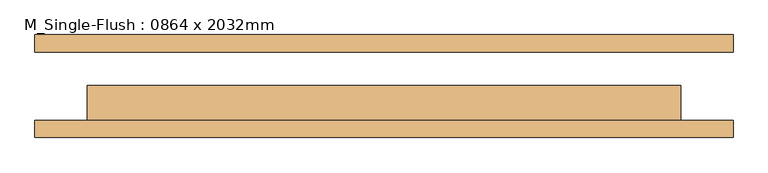
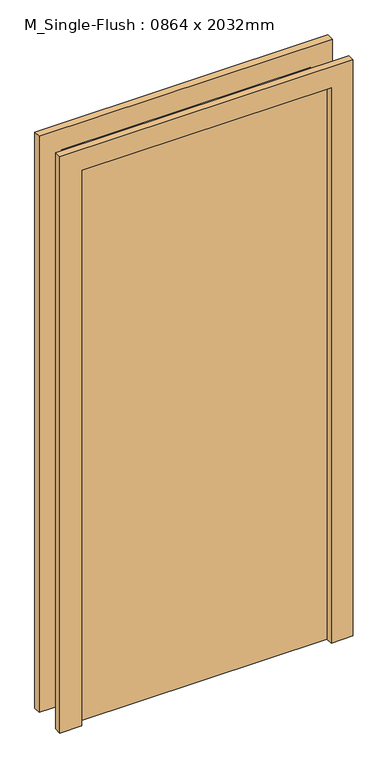
"""IFC4 building model written with IfcOpenShell, lengths in millimetres: door geometry, M_Single-Flush : 0864 x 2032mm."""

import ifcopenshell
import ifcopenshell.guid

model = None  # the IFC model being written
_history = None  # IfcOwnerHistory: only IFC2X3 demands one
_inside = {}  # id of a spatial element -> (the spatial element, [elements in it])
_under = {}  # id of a project, library or spatial element -> (it, [spatial elements below it])
_declared = {}  # id of a project -> (the project, [libraries it declares])
_typed = {}  # id of a type object -> (the type object, [elements of that type])
_made_of = {}  # id of a material, layer set ... -> (it, [elements and type objects made of it])


def new_model(schema):
    """Start an empty IFC model of exactly this schema.

    Asked for "IFC4X3", IfcOpenShell would pick the latest addendum, in which some entities
    have other attributes; the version numbers below select the first issue.
    IFC2X3 requires an IfcOwnerHistory on every rooted entity: one is made here for all.
    """
    global model, _history
    if schema == "IFC4X3":
        model = ifcopenshell.file(schema_version=(4, 3, 0, 0))
    else:
        model = ifcopenshell.file(schema=schema)
    _inside.clear()
    _under.clear()
    _declared.clear()
    _typed.clear()
    _made_of.clear()
    _history = None
    if model.schema == "IFC2X3":
        org = make("IfcOrganization", Name="unknown")
        user = make(
            "IfcPersonAndOrganization",
            ThePerson=make("IfcPerson", FamilyName="unknown"),
            TheOrganization=org,
        )
        app = make(
            "IfcApplication",
            ApplicationDeveloper=org,
            Version="unknown",
            ApplicationFullName="unknown",
            ApplicationIdentifier="unknown",
        )
        _history = make(
            "IfcOwnerHistory",
            OwningUser=user,
            OwningApplication=app,
            ChangeAction="ADDED",
            CreationDate=0,
        )
    return model


def make(cls, **values):
    """One entity of the class cls with the attributes given. An attribute that is None is left unset."""
    return model.create_entity(
        cls, **{name: value for name, value in values.items() if value is not None}
    )


def rooted(cls, **values):
    """An entity with a GlobalId (a new one), such as an element, a storey or a relation."""
    return make(cls, GlobalId=ifcopenshell.guid.new(), OwnerHistory=_history, **values)


def si_unit(unit_type, name, prefix=None):
    """IfcSIUnit, for example si_unit("LENGTHUNIT", "METRE", prefix="MILLI")."""
    return make("IfcSIUnit", UnitType=unit_type, Prefix=prefix, Name=name)


def assignment(units):
    """IfcUnitAssignment: the units of a project."""
    return None if units is None else make("IfcUnitAssignment", Units=units)


def point(xyz):
    """IfcCartesianPoint."""
    return None if xyz is None else make("IfcCartesianPoint", Coordinates=xyz)


def direction(xyz):
    """IfcDirection."""
    return None if xyz is None else make("IfcDirection", DirectionRatios=xyz)


def frame(location, z_axis=None, x_axis=None):
    """IfcAxis2Placement3D, a coordinate frame: its origin and axes. An axis left out is left unset."""
    return make(
        "IfcAxis2Placement3D",
        Location=point(location),
        Axis=direction(z_axis),
        RefDirection=direction(x_axis),
    )


def origin():
    """The frame at (0, 0, 0) with its axes left unset."""
    return frame((0.0, 0.0, 0.0))


def origin_with_axes():
    """The frame at (0, 0, 0) with the z axis (0, 0, 1) and the x axis (1, 0, 0) written out."""
    return frame((0.0, 0.0, 0.0), z_axis=(0.0, 0.0, 1.0), x_axis=(1.0, 0.0, 0.0))


def place(relative_to, where):
    """IfcLocalPlacement: puts the frame where relative to a parent placement (None: the world)."""
    return make(
        "IfcLocalPlacement", PlacementRelTo=relative_to, RelativePlacement=where
    )


def context(
    kind, dimensions, precision=None, world=None, true_north=None, identifier=None
):
    """IfcGeometricRepresentationContext, for example the 3D "Model" context."""
    return make(
        "IfcGeometricRepresentationContext",
        ContextIdentifier=identifier,
        ContextType=kind,
        CoordinateSpaceDimension=dimensions,
        Precision=precision,
        WorldCoordinateSystem=world,
        TrueNorth=true_north,
    )


def project(units=None, contexts=None):
    """IfcProject with its units and contexts."""
    return rooted(
        "IfcProject",
        Name="project",
        RepresentationContexts=contexts,
        UnitsInContext=assignment(units),
    )


def spatial(cls, under=None, at=None, **own):
    """A site, building, storey or space (cls), placed at a placement, below another one or the project."""
    s = rooted(cls, ObjectPlacement=at, **own)
    if under is not None:
        _under.setdefault(under.id(), (under, []))[1].append(s)
    return s


def polyline(points):
    """IfcPolyline through the points."""
    return make("IfcPolyline", Points=[point(p) for p in points])


def outline(outer, holes=None, kind="AREA"):
    """IfcArbitraryClosedProfileDef: a profile drawn as a closed curve; with holes, ...WithVoids."""
    if holes is None:
        return make("IfcArbitraryClosedProfileDef", ProfileType=kind, OuterCurve=outer)
    return make(
        "IfcArbitraryProfileDefWithVoids",
        ProfileType=kind,
        OuterCurve=outer,
        InnerCurves=holes,
    )


def extrude(swept, where, along, depth):
    """IfcExtrudedAreaSolid: the profile swept, set in the frame where, extruded along a direction by depth."""
    return make(
        "IfcExtrudedAreaSolid",
        SweptArea=swept,
        Position=where,
        ExtrudedDirection=direction(along),
        Depth=depth,
    )


def shape(context_of_items, identifier, shape_type, items):
    """IfcShapeRepresentation: the items that make up one representation, for example the "Body"."""
    return make(
        "IfcShapeRepresentation",
        ContextOfItems=context_of_items,
        RepresentationIdentifier=identifier,
        RepresentationType=shape_type,
        Items=items,
    )


def source(mapping_origin, context_of_items, identifier, shape_type, items):
    """IfcRepresentationMap: a shape defined once, which mapped items show again and again."""
    return make(
        "IfcRepresentationMap",
        MappingOrigin=mapping_origin,
        MappedRepresentation=shape(context_of_items, identifier, shape_type, items),
    )


def transform(
    local_origin,
    x_axis=None,
    y_axis=None,
    z_axis=None,
    scale=None,
    scale2=None,
    scale3=None,
    uniform=True,
):
    """IfcCartesianTransformationOperator3D, or its non-uniform kind. x_axis, y_axis, z_axis: its Axis1, 2, 3."""
    if uniform:
        return make(
            "IfcCartesianTransformationOperator3D",
            Axis1=direction(x_axis),
            Axis2=direction(y_axis),
            LocalOrigin=point(local_origin),
            Scale=scale,
            Axis3=direction(z_axis),
        )
    return make(
        "IfcCartesianTransformationOperator3DnonUniform",
        Axis1=direction(x_axis),
        Axis2=direction(y_axis),
        LocalOrigin=point(local_origin),
        Scale=scale,
        Axis3=direction(z_axis),
        Scale2=scale2,
        Scale3=scale3,
    )


def mapped(mapping_source, mapping_target):
    """IfcMappedItem: shows the shape of a source again, moved by a transform."""
    return make(
        "IfcMappedItem", MappingSource=mapping_source, MappingTarget=mapping_target
    )


def made_of(thing, what):
    """Note that an element or type object is made of a material, layer set ...; save() writes the relation."""
    if what is not None:
        _made_of.setdefault(what.id(), (what, []))[1].append(thing)
    return thing


def element(
    cls,
    number,
    at=None,
    inside=None,
    cuts=None,
    type_object=None,
    material=None,
    context=None,
    identifier="Body",
    shape_type=None,
    held_by="IfcProductDefinitionShape",
    body=None,
    shapes=None,
    **own,
):
    """One element of the class cls, such as IfcWall. Its Tag is "e" and its number.

    at: its placement. inside: the storey or other place that contains it. cuts: it is an
    opening in that element (IfcRelVoidsElement). A single representation is given by context,
    identifier, shape_type and body (its items); several are given by shapes. held_by: the class
    of the entity that holds the representations. save() writes the other relations.
    """
    e = rooted(cls, Tag="e%d" % number, ObjectPlacement=at, **own)
    if body is not None:
        shapes = [shape(context, identifier, shape_type, body)]
    if shapes is not None:
        e.Representation = make(held_by, Representations=shapes)
    if inside is not None:
        _inside.setdefault(inside.id(), (inside, []))[1].append(e)
    if cuts is not None:
        rooted(
            "IfcRelVoidsElement", RelatingBuildingElement=cuts, RelatedOpeningElement=e
        )
    if type_object is not None:
        _typed.setdefault(type_object.id(), (type_object, []))[1].append(e)
    return made_of(e, material)


def aggregate(whole, parts):
    """IfcRelAggregates: a whole, such as a stair, and the parts it consists of."""
    return rooted("IfcRelAggregates", RelatingObject=whole, RelatedObjects=parts)


def save(model, path):
    """Write the relations noted so far, then the file.

    IfcRelAggregates (storeys below a building ...), IfcRelContainedInSpatialStructure (elements
    in a storey), IfcRelDefinesByType, IfcRelAssociatesMaterial and IfcRelDeclares: one each for
    every whole, place, type object, material and project.
    """
    for whole, parts in _under.values():
        aggregate(whole, parts)
    for where, things in _inside.values():
        rooted(
            "IfcRelContainedInSpatialStructure",
            RelatedElements=things,
            RelatingStructure=where,
        )
    for kind, things in _typed.values():
        rooted("IfcRelDefinesByType", RelatedObjects=things, RelatingType=kind)
    for what, things in _made_of.values():
        rooted("IfcRelAssociatesMaterial", RelatedObjects=things, RelatingMaterial=what)
    for by, libraries in _declared.values():
        rooted("IfcRelDeclares", RelatingContext=by, RelatedDefinitions=libraries)
    model.write(path)


def m_single_flush_0864_x_2032mm_0d7903e5(model_context):
    return source(origin(), model_context, "Body", "SweptSolid", [
        extrude(outline(polyline([(2108.0, -508.0), (0.0, -508.0), (0.0, -432.0), (2032.0, -432.0), (2032.0, 432.0), (0.0, 432.0), (0.0, 508.0), (2108.0, 508.0), (2108.0, -508.0)])), frame((0.0, -75.0, 0.0), z_axis=(0.0, 1.0, 0.0), x_axis=(0.0, 0.0, 1.0)), (0.0, 0.0, 1.0), 25.0),
        extrude(outline(polyline([(2108.0, 508.0), (2108.0, -508.0), (0.0, -508.0), (0.0, -432.0), (2032.0, -432.0), (2032.0, 432.0), (0.0, 432.0), (0.0, 508.0), (2108.0, 508.0)])), frame((0.0, 50.0, 0.0), z_axis=(0.0, 1.0, 0.0), x_axis=(0.0, 0.0, 1.0)), (0.0, 0.0, 1.0), 25.0),
        extrude(outline(polyline([(432.0, 1.0), (432.0, -50.0), (-432.0, -50.0), (-432.0, 1.0), (432.0, 1.0)])), origin_with_axes(), (0.0, 0.0, 1.0), 2032.0),
    ])


if __name__ == "__main__":
    model = new_model("IFC4")
    model_context = context("Model", 3, world=origin())
    ifc_project = project(units=[si_unit("LENGTHUNIT", "METRE", prefix="MILLI")], contexts=[model_context])
    site = spatial("IfcSite", under=ifc_project)
    building = spatial("IfcBuilding", under=site)
    placement = place(None, origin())
    m_single_flush_0864_x_2032mm_shape = m_single_flush_0864_x_2032mm_0d7903e5(model_context)
    element("IfcDoor", 1, ObjectType="M_Single-Flush : 0864 x 2032mm", at=placement, inside=building, context=model_context, shape_type="MappedRepresentation", body=[
        mapped(m_single_flush_0864_x_2032mm_shape, transform((0.0, 0.0, 0.0), x_axis=(1.0, 0.0, 0.0), y_axis=(0.0, 1.0, 0.0), z_axis=(0.0, 0.0, 1.0))),
    ])
    save(model, "model.ifc")

# Revit data of these elements
# Project information
#   Organization Name = "SHV"
#   Building Name = "Pere Valencia"
#   Author = "Ian Salter"
#   Project Issue Date = "Issue Date"
#   Project Status = "Project  Status"
#   Client Name = "Ian Salter"
#   Project Address = "## Street\nCity, State  Zip"
#   Project Name = "Project Name"
#   Project Number = "Project  Number"
# Type "M_Single-Flush : 0864 x 2032mm"
#   Type Mark = "21"
#   Thickness = 5.1 cm
#   Height = 203.2 cm
#   Trim Projection Ext = 2.5 cm
#   Trim Projection Int = 2.5 cm
#   Trim Width = 7.6 cm
#   Width = 86.4 cm
#   Door Material = Door - Panel
#   Frame Material = Door - Frame
#   Function = (empty or 0)
#   Wall Closure = (empty or 0)
# Element 1 (IfcDoor, "M_Single-Flush : 0864 x 2032mm")
#   Materials on its faces: "Door - Frame", "Door - Panel"
# Materials
#   "Door - Panel": class "Wood", colour RGB 114 82 51, transparency 0
#   "Door - Frame": class "Miscellaneous", colour RGB 153 76 43, transparency 0
